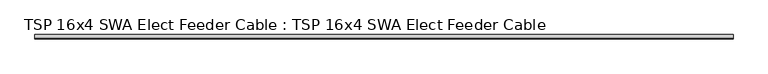
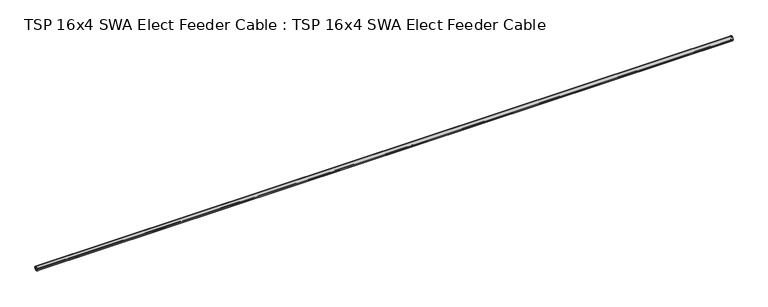
"""IFC4 building model written with IfcOpenShell, lengths in millimetres: proxy geometry, TSP 16x4 SWA Elect Feeder Cable : TSP 16x4 SWA Elect Feeder Cable."""

from ifc_helpers import new_model, si_unit, point, frame, frame_2d, origin, origin_2d, place, context, project, spatial, circle_curve, trimmed, segment, composite_curve, outline, extrude, source, transform, mapped, element, save


def tsp_16x4_swa_elect_feeder_cable_tsp_16x4_swa_elect_feeder_87b5e402(model_context):
    return source(origin(), model_context, "Body", "SweptSolid", [
        extrude(outline(composite_curve([segment(trimmed(circle_curve(origin_2d(), 30.0), [point((-30.0, 0.0))], [point((30.0, 0.0))], False, "CARTESIAN"), True, "CONTINUOUS"), segment(trimmed(circle_curve(origin_2d(), 30.0), [point((30.0, 0.0))], [point((-30.0, 0.0))], False, "CARTESIAN"), True, "CONTINUOUS")], self_intersect=False), holes=[composite_curve([segment(trimmed(circle_curve(origin_2d(), 27.0), [point((-27.0, 0.0))], [point((27.0, 0.0))], True, "CARTESIAN"), True, "CONTINUOUS"), segment(trimmed(circle_curve(origin_2d(), 27.0), [point((27.0, 0.0))], [point((-27.0, 0.0))], True, "CARTESIAN"), True, "CONTINUOUS")], self_intersect=False)]), frame((0.0, 0.0, 0.0), z_axis=(1.0, 0.0, 0.0), x_axis=(0.0, 1.0, 0.0)), (0.0, 0.0, 1.0), 9624.5440731),
        extrude(outline(composite_curve([segment(trimmed(circle_curve(frame_2d((11.691343, 10.1)), 8.0), [point((3.691343, 10.1))], [point((19.691343, 10.1))], False, "CARTESIAN"), True, "CONTINUOUS"), segment(trimmed(circle_curve(frame_2d((11.691343, 10.1)), 8.0), [point((19.691343, 10.1))], [point((3.691343, 10.1))], False, "CARTESIAN"), True, "CONTINUOUS")], self_intersect=False)), frame((0.0, 0.0, 0.0), z_axis=(1.0, 0.0, 0.0), x_axis=(0.0, 1.0, 0.0)), (0.0, 0.0, 1.0), 9624.5440731),
        extrude(outline(composite_curve([segment(trimmed(circle_curve(frame_2d((-11.691343, 10.1)), 8.0), [point((-19.691343, 10.1))], [point((-3.691343, 10.1))], False, "CARTESIAN"), True, "CONTINUOUS"), segment(trimmed(circle_curve(frame_2d((-11.691343, 10.1)), 8.0), [point((-3.691343, 10.1))], [point((-19.691343, 10.1))], False, "CARTESIAN"), True, "CONTINUOUS")], self_intersect=False)), frame((0.0, 0.0, 0.0), z_axis=(1.0, 0.0, 0.0), x_axis=(0.0, 1.0, 0.0)), (0.0, 0.0, 1.0), 9624.5440731),
        extrude(outline(composite_curve([segment(trimmed(circle_curve(frame_2d((-11.691343, -10.1)), 8.0), [point((-19.691343, -10.1))], [point((-3.691343, -10.1))], False, "CARTESIAN"), True, "CONTINUOUS"), segment(trimmed(circle_curve(frame_2d((-11.691343, -10.1)), 8.0), [point((-3.691343, -10.1))], [point((-19.691343, -10.1))], False, "CARTESIAN"), True, "CONTINUOUS")], self_intersect=False)), frame((0.0, 0.0, 0.0), z_axis=(1.0, 0.0, 0.0), x_axis=(0.0, 1.0, 0.0)), (0.0, 0.0, 1.0), 9624.5440731),
        extrude(outline(composite_curve([segment(trimmed(circle_curve(frame_2d((11.691343, -10.1)), 8.0), [point((3.691343, -10.1))], [point((19.691343, -10.1))], False, "CARTESIAN"), True, "CONTINUOUS"), segment(trimmed(circle_curve(frame_2d((11.691343, -10.1)), 8.0), [point((19.691343, -10.1))], [point((3.691343, -10.1))], False, "CARTESIAN"), True, "CONTINUOUS")], self_intersect=False)), frame((0.0, 0.0, 0.0), z_axis=(1.0, 0.0, 0.0), x_axis=(0.0, 1.0, 0.0)), (0.0, 0.0, 1.0), 9624.5440731),
        extrude(outline(composite_curve([segment(trimmed(circle_curve(origin_2d(), 27.0), [point((27.0, 0.0))], [point((-27.0, 0.0))], False, "CARTESIAN"), True, "CONTINUOUS"), segment(trimmed(circle_curve(origin_2d(), 27.0), [point((-27.0, 0.0))], [point((27.0, 0.0))], False, "CARTESIAN"), True, "CONTINUOUS")], self_intersect=False), holes=[composite_curve([segment(trimmed(circle_curve(frame_2d((-11.691343, 10.1)), 8.0), [point((-3.691343, 10.1))], [point((-19.691343, 10.1))], True, "CARTESIAN"), True, "CONTINUOUS"), segment(trimmed(circle_curve(frame_2d((-11.691343, 10.1)), 8.0), [point((-19.691343, 10.1))], [point((-3.691343, 10.1))], True, "CARTESIAN"), True, "CONTINUOUS")], self_intersect=False), composite_curve([segment(trimmed(circle_curve(frame_2d((11.691343, 10.1)), 8.0), [point((3.691343, 10.1))], [point((19.691343, 10.1))], True, "CARTESIAN"), True, "CONTINUOUS"), segment(trimmed(circle_curve(frame_2d((11.691343, 10.1)), 8.0), [point((19.691343, 10.1))], [point((3.691343, 10.1))], True, "CARTESIAN"), True, "CONTINUOUS")], self_intersect=False), composite_curve([segment(trimmed(circle_curve(frame_2d((-11.691343, -10.15)), 8.0), [point((-19.691343, -10.15))], [point((-3.691343, -10.15))], True, "CARTESIAN"), True, "CONTINUOUS"), segment(trimmed(circle_curve(frame_2d((-11.691343, -10.15)), 8.0), [point((-3.691343, -10.15))], [point((-19.691343, -10.15))], True, "CARTESIAN"), True, "CONTINUOUS")], self_intersect=False), composite_curve([segment(trimmed(circle_curve(frame_2d((11.691343, -10.15)), 8.0), [point((3.691343, -10.15))], [point((19.691343, -10.15))], True, "CARTESIAN"), True, "CONTINUOUS"), segment(trimmed(circle_curve(frame_2d((11.691343, -10.15)), 8.0), [point((19.691343, -10.15))], [point((3.691343, -10.15))], True, "CARTESIAN"), True, "CONTINUOUS")], self_intersect=False)]), frame((0.0, 0.0, 0.0), z_axis=(1.0, 0.0, 0.0), x_axis=(0.0, 1.0, 0.0)), (0.0, 0.0, 1.0), 9624.5440731),
    ])


if __name__ == "__main__":
    model = new_model("IFC4")
    model_context = context("Model", 3, world=origin())
    ifc_project = project(units=[si_unit("LENGTHUNIT", "METRE", prefix="MILLI")], contexts=[model_context])
    site = spatial("IfcSite", under=ifc_project)
    building = spatial("IfcBuilding", under=site)
    placement = place(None, origin())
    tsp_16x4_swa_elect_feeder_cable_tsp_16x4_swa_elect_feeder_shape = tsp_16x4_swa_elect_feeder_cable_tsp_16x4_swa_elect_feeder_87b5e402(model_context)
    element("IfcBuildingElementProxy", 1, Name="TSP 16x4 SWA Elect Feeder Cable : TSP 16x4 SWA Elect Feeder Cable", ObjectType="TSP 16x4 SWA Elect Feeder Cable : TSP 16x4 SWA Elect Feeder Cable", at=placement, inside=building, context=model_context, shape_type="MappedRepresentation", body=[
        mapped(tsp_16x4_swa_elect_feeder_cable_tsp_16x4_swa_elect_feeder_shape, transform((0.0, 0.0, 0.0), x_axis=(1.0, 0.0, 0.0), y_axis=(0.0, 1.0, 0.0), z_axis=(0.0, 0.0, 1.0))),
    ])
    save(model, "model.ifc")

# Revit data of these elements
# Type "TSP 16x4 SWA Elect Feeder Cable : TSP 16x4 SWA Elect Feeder Cable"
#   Model = "TSP_ELECSC164"
#   built-in parameter 1001306 [instance default] = 5.24934 (stored number, unit not read)
#   Cable Length [instance default] = 1600 mm
#   Default Elevation = 0
# Element 1 (IfcBuildingElementProxy, "TSP 16x4 SWA Elect Feeder Cable : TSP 16x4 SWA Elect Feeder Cable")
#   built-in parameter 1001306 = 31.5766 (stored number, unit not read)
#   Cable Length = 9624.544 mm
#   Materials on its faces: "Cellulose Fill", "Copper", "Laminate, Red, Matte"
# Materials
#   "Cellulose Fill": class "Generic", colour RGB 0 0 0, transparency 0, Description = "Cellulose loose fill", Cost = 0
#   "Copper": class "Metal", colour RGB 0 0 0, transparency 0, Description = "Copper, matte finish", Cost = 0
#   "Laminate, Red, Matte": class "Plastic", colour RGB 255 0 0, transparency 0, Description = "Plastic Laminate - Red, Matte", Cost = 0
